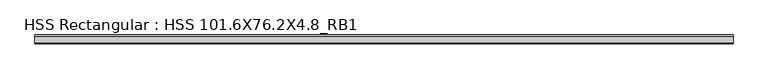
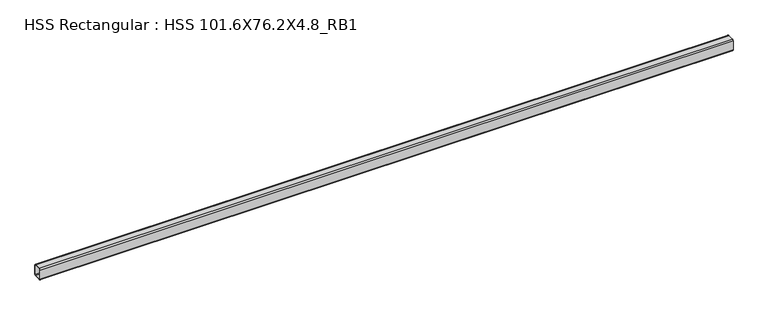
"""IFC4 building model written with IfcOpenShell, lengths in millimetres: beam geometry, HSS Rectangular : HSS 101.6X76.2X4.8_RB1."""

from ifc_helpers import new_model, si_unit, point, frame, frame_2d, origin, place, context, project, spatial, polyline, circle_curve, trimmed, segment, composite_curve, outline, extrude, source, transform, mapped, element, save


def hss_rectangular_hss_101_6x76_2x4_8_rb1_c80bc8ef(model_context):
    return source(origin(), model_context, "Body", "SweptSolid", [
        extrude(outline(composite_curve([segment(polyline([(38.1, 41.275), (38.1, -41.275)]), True, "CONTINUOUS"), segment(trimmed(circle_curve(frame_2d((28.575, -41.275)), 9.525), [point((38.1, -41.275))], [point((28.575, -50.8))], False, "CARTESIAN"), True, "CONTINUOUS"), segment(polyline([(28.575, -50.8), (-28.575, -50.8)]), True, "CONTINUOUS"), segment(trimmed(circle_curve(frame_2d((-28.575, -41.275)), 9.525), [point((-28.575, -50.8))], [point((-38.1, -41.275))], False, "CARTESIAN"), True, "CONTINUOUS"), segment(polyline([(-38.1, -41.275), (-38.1, 41.275)]), True, "CONTINUOUS"), segment(trimmed(circle_curve(frame_2d((-28.575, 41.275)), 9.525), [point((-38.1, 41.275))], [point((-28.575, 50.8))], False, "CARTESIAN"), True, "CONTINUOUS"), segment(polyline([(-28.575, 50.8), (28.575, 50.8)]), True, "CONTINUOUS"), segment(trimmed(circle_curve(frame_2d((28.575, 41.275)), 9.525), [point((28.575, 50.8))], [point((38.1, 41.275))], False, "CARTESIAN"), True, "CONTINUOUS")], self_intersect=False), holes=[composite_curve([segment(trimmed(circle_curve(frame_2d((-28.575, 41.275)), 4.7625), [point((-28.575, 46.0375))], [point((-33.3375, 41.275))], True, "CARTESIAN"), True, "CONTINUOUS"), segment(polyline([(-33.3375, 41.275), (-33.3375, -41.275)]), True, "CONTINUOUS"), segment(trimmed(circle_curve(frame_2d((-28.575, -41.275)), 4.7625), [point((-33.3375, -41.275))], [point((-28.575, -46.0375))], True, "CARTESIAN"), True, "CONTINUOUS"), segment(polyline([(-28.575, -46.0375), (28.575, -46.0375)]), True, "CONTINUOUS"), segment(trimmed(circle_curve(frame_2d((28.575, -41.275)), 4.7625), [point((28.575, -46.0375))], [point((33.3375, -41.275))], True, "CARTESIAN"), True, "CONTINUOUS"), segment(polyline([(33.3375, -41.275), (33.3375, 41.275)]), True, "CONTINUOUS"), segment(trimmed(circle_curve(frame_2d((28.575, 41.275)), 4.7625), [point((33.3375, 41.275))], [point((28.575, 46.0375))], True, "CARTESIAN"), True, "CONTINUOUS"), segment(polyline([(28.575, 46.0375), (-28.575, 46.0375)]), True, "CONTINUOUS")], self_intersect=False)]), frame((-7482.761, 0.0, 0.0), z_axis=(1.0, 0.0, 0.0), x_axis=(0.0, 1.0, 0.0)), (0.0, 0.0, 1.0), 6014.511),
    ])


if __name__ == "__main__":
    model = new_model("IFC4")
    model_context = context("Model", 3, world=origin())
    ifc_project = project(units=[si_unit("LENGTHUNIT", "METRE", prefix="MILLI")], contexts=[model_context])
    site = spatial("IfcSite", under=ifc_project)
    building = spatial("IfcBuilding", under=site)
    placement = place(None, origin())
    hss_rectangular_hss_101_6x76_2x4_8_rb1_shape = hss_rectangular_hss_101_6x76_2x4_8_rb1_c80bc8ef(model_context)
    element("IfcBeam", 1, ObjectType="HSS Rectangular : HSS 101.6X76.2X4.8_RB1", at=placement, inside=building, context=model_context, shape_type="MappedRepresentation", body=[
        mapped(hss_rectangular_hss_101_6x76_2x4_8_rb1_shape, transform((0.0, 0.0, 0.0), x_axis=(1.0, 0.0, 0.0), y_axis=(0.0, 1.0, 0.0), z_axis=(0.0, 0.0, 1.0))),
    ])
    save(model, "model.ifc")

# Revit data of these elements
# Type "HSS Rectangular : HSS 101.6X76.2X4.8_RB1"
#   Section Name Key = "HSS 4X3X3/16"
#   Assembly Code = "B10"
#   Width = 7.62 cm
#   Wall Nominal Thickness = 0.4763 cm
#   Wall Design Thickness = 0.442 cm
#   Torsional Moment of Inertia = 260.561 cm⁴
#   Torsional Modulus = 61.2876 cm³
#   Section Area = 14.4516 cm²
#   Plastic Modulus weak axis = 40.3122 cm³
#   Plastic Modulus strong axis = 49.1612 cm³
#   Perimeter = 0.881482 m²/m
#   Outer Fillet = 0.9525 cm
#   Nominal Weight = 12.1285 kgf/m
#   Moment of Inertia weak axis = 131.529 cm⁴
#   Moment of Inertia strong axis = 205.202 cm⁴
#   Inner Fillet = 0.4763 cm
#   Height = 10.16 cm
#   Elastic Modulus weak axis = 34.4128 cm³
#   Elastic Modulus strong axis = 40.476 cm³
#   Centroid Vertical = 5.08 cm
#   Centroid Horizontal = 3.81 cm
#   Length [instance default] = 1524 mm
#   Structural Material [instance default] = Steel ASTM A500, Grade B, Rectangular and Square
#   Principal Axes Angle = 0
# Element 1 (IfcBeam, "HSS Rectangular : HSS 101.6X76.2X4.8_RB1")
#   Structural Material = Steel ASTM A992
#   Materials on its faces: "Steel ASTM A992"
# Materials
#   "Steel ASTM A500, Grade B, Rectangular and Square": class "Metal", colour RGB 199 199 199, transparency 0, Description = "Carbon steel", Cost = 0
#   "Steel ASTM A992": class "Metal", colour RGB 199 199 199, transparency 0, Description = "Structural steel 50ksi", Cost = 0
